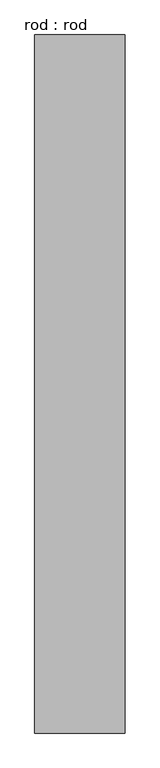
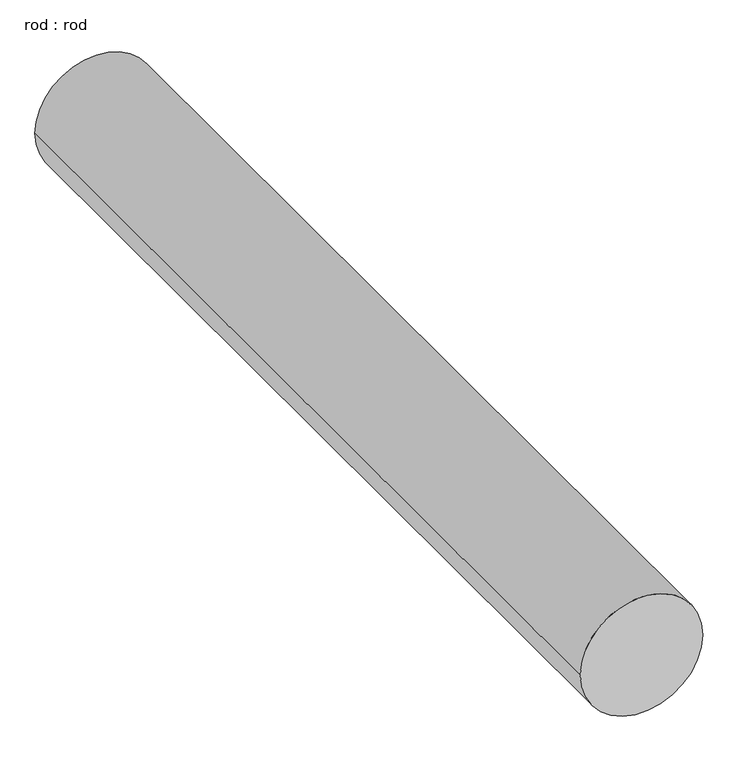
"""IFC4 building model written with IfcOpenShell, lengths in millimetres: proxy geometry, rod : rod."""

from ifc_helpers import new_model, si_unit, point, frame, frame_2d, origin, place, context, project, spatial, circle_curve, trimmed, segment, composite_curve, outline, extrude, source, transform, mapped, element, save


def rod_rod_64a08bc0(model_context):
    return source(origin(), model_context, "Body", "SweptSolid", [
        extrude(outline(composite_curve([segment(trimmed(circle_curve(frame_2d((0.0108462, 0.0)), 200.0), [point((0.0108462, 200.0))], [point((0.0108462, -200.0))], False, "CARTESIAN"), True, "CONTINUOUS"), segment(trimmed(circle_curve(frame_2d((0.0108462, 0.0)), 200.0), [point((0.0108462, -200.0))], [point((0.0108462, 200.0))], False, "CARTESIAN"), True, "CONTINUOUS")], self_intersect=False)), frame((0.0, 2549.8714725, 0.0), z_axis=(0.0, 1.0, 0.0), x_axis=(0.0, 0.0, 1.0)), (0.0, 0.0, 1.0), 3085.7142857),
    ])


if __name__ == "__main__":
    model = new_model("IFC4")
    model_context = context("Model", 3, world=origin())
    ifc_project = project(units=[si_unit("LENGTHUNIT", "METRE", prefix="MILLI")], contexts=[model_context])
    site = spatial("IfcSite", under=ifc_project)
    building = spatial("IfcBuilding", under=site)
    placement = place(None, origin())
    rod_rod_shape = rod_rod_64a08bc0(model_context)
    element("IfcBuildingElementProxy", 1, Name="rod : rod", ObjectType="rod : rod", at=placement, inside=building, context=model_context, shape_type="MappedRepresentation", body=[
        mapped(rod_rod_shape, transform((0.0, 0.0, 0.0), x_axis=(1.0, 0.0, 0.0), y_axis=(0.0, 1.0, 0.0), z_axis=(0.0, 0.0, 1.0))),
    ])
    save(model, "model.ifc")

# Revit data of these elements
# Type "rod : rod"
#   Default Elevation = 0
